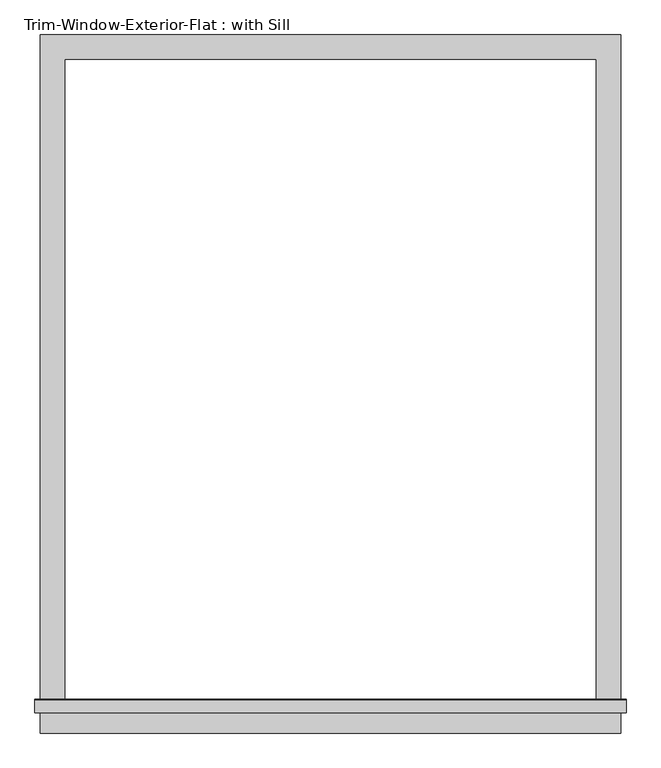
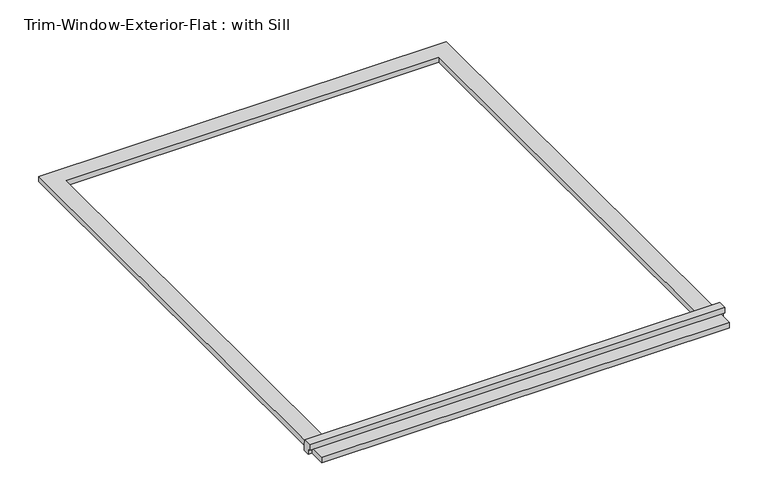
"""IFC4 building model written with IfcOpenShell, lengths in millimetres: proxy geometry, Trim-Window-Exterior-Flat : with Sill."""

from ifc_helpers import new_model, si_unit, frame, origin, origin_with_axes, place, context, project, spatial, polyline, outline, extrude, source, transform, mapped, element, save


def trim_window_exterior_flat_with_sill_e43f37a2(model_context):
    return source(origin(), model_context, "Body", "SweptSolid", [
        extrude(outline(polyline([(679.45, -1520.7823709), (679.45, -1577.9323709), (-679.45, -1577.9323709), (-679.45, -1520.7823709), (679.45, -1520.7823709)])), origin_with_axes(), (0.0, 0.0, 1.0), 19.05),
        extrude(outline(polyline([(-1530.35, 38.1), (-1501.0580645, 38.1), (-1498.6, 19.05), (-1498.6, 0.0), (-1520.7823709, 0.0), (-1520.7823709, 19.05), (-1530.35, 19.05), (-1530.35, 38.1)])), frame((-692.15, 0.0, 0.0), z_axis=(1.0, 0.0, 0.0), x_axis=(0.0, 1.0, 0.0)), (0.0, 0.0, 1.0), 1384.3),
        extrude(outline(polyline([(-679.45, 57.15), (679.45, 57.15), (679.45, -1498.6), (622.3, -1498.6), (622.3, 0.0), (-622.3, 0.0), (-622.3, -1498.6), (-679.45, -1498.6), (-679.45, 57.15)])), origin_with_axes(), (0.0, 0.0, 1.0), 19.05),
    ])


if __name__ == "__main__":
    model = new_model("IFC4")
    model_context = context("Model", 3, world=origin())
    ifc_project = project(units=[si_unit("LENGTHUNIT", "METRE", prefix="MILLI")], contexts=[model_context])
    site = spatial("IfcSite", under=ifc_project)
    building = spatial("IfcBuilding", under=site)
    placement = place(None, origin())
    trim_window_exterior_flat_with_sill_shape = trim_window_exterior_flat_with_sill_e43f37a2(model_context)
    element("IfcBuildingElementProxy", 1, Name="Trim-Window-Exterior-Flat : with Sill", ObjectType="Trim-Window-Exterior-Flat : with Sill", at=placement, inside=building, context=model_context, shape_type="MappedRepresentation", body=[
        mapped(trim_window_exterior_flat_with_sill_shape, transform((0.0, 0.0, 0.0), x_axis=(1.0, 0.0, 0.0), y_axis=(0.0, 1.0, 0.0), z_axis=(0.0, 0.0, 1.0))),
    ])
    save(model, "model.ifc")

# Revit data of these elements
# Type "Trim-Window-Exterior-Flat : with Sill"
#   Trim Width = 0' - 2 1/4"
#   Trim Thickness_Picture Frame = 0' - 1 1/4"
#   Trim Thickness_with Sill = 0' - 0 3/4"
#   Sill Thickness = 0' - 1 1/4"
#   Opening Width [instance default] = 2' - 0"
#   Opening Height [instance default] = 3' - 0"
#   Default Elevation = 4' - 0"
#   Sill = yes
#   Picture Frame = no
#   Trim Material [instance default] = none
# Element 1 (IfcBuildingElementProxy, "Trim-Window-Exterior-Flat : with Sill")
#   Opening Width = 4' - 1"
#   Opening Height = 4' - 11"
#   Trim Material = 1X WOOD COMPOSITE TRIM
#   Materials on its faces: "1X WOOD COMPOSITE TRIM"
# Materials
#   "1X WOOD COMPOSITE TRIM": class "Generic", colour RGB 88 61 61, transparency 0, Cost = 0
